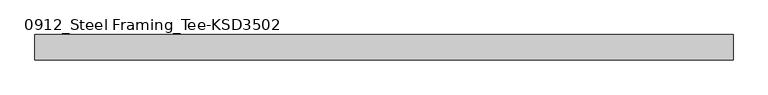
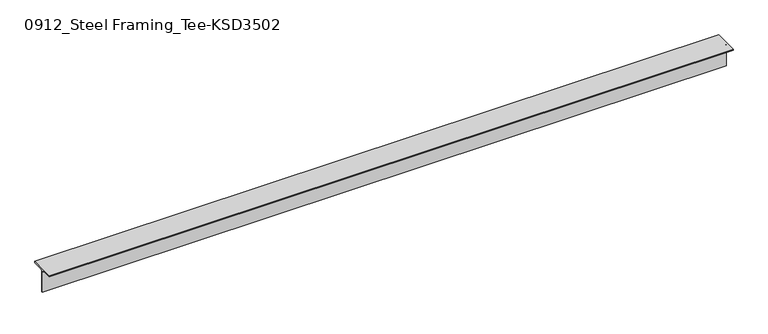
"""IFC4 building model written with IfcOpenShell, lengths in millimetres: member geometry, 0912_Steel Framing_Tee-KSD3502 : H_SB_ASB_CT-150x150x6.5x9."""

from ifc_helpers import new_model, si_unit, point, frame, frame_2d, origin, place, context, project, spatial, polyline, circle_curve, trimmed, segment, composite_curve, outline, extrude, source, transform, mapped, element, save


def member_0912_steel_framing_tee_ksd3502_323286f3(model_context):
    return source(origin(), model_context, "Body", "SweptSolid", [
        extrude(outline(composite_curve([segment(polyline([(-75.0, 75.0), (75.0, 75.0), (75.0, 66.0), (16.25, 66.0)]), True, "CONTINUOUS"), segment(trimmed(circle_curve(frame_2d((16.25, 53.0)), 13.0), [point((16.25, 66.0))], [point((3.25, 53.0))], True, "CARTESIAN"), True, "CONTINUOUS"), segment(polyline([(3.25, 53.0), (3.25, -75.0), (-3.25, -75.0), (-3.25, 53.0)]), True, "CONTINUOUS"), segment(trimmed(circle_curve(frame_2d((-16.25, 53.0)), 13.0), [point((-3.25, 53.0))], [point((-16.25, 66.0))], True, "CARTESIAN"), True, "CONTINUOUS"), segment(polyline([(-16.25, 66.0), (-75.0, 66.0), (-75.0, 75.0)]), True, "CONTINUOUS")], self_intersect=False)), frame((-2059.45, 0.0, 0.0), z_axis=(1.0, 0.0, 0.0), x_axis=(0.0, 1.0, 0.0)), (0.0, 0.0, 1.0), 4153.3),
    ])


if __name__ == "__main__":
    model = new_model("IFC4")
    model_context = context("Model", 3, world=origin())
    ifc_project = project(units=[si_unit("LENGTHUNIT", "METRE", prefix="MILLI")], contexts=[model_context])
    site = spatial("IfcSite", under=ifc_project)
    building = spatial("IfcBuilding", under=site)
    placement = place(None, origin())
    member_0912_steel_framing_tee_ksd3502_shape = member_0912_steel_framing_tee_ksd3502_323286f3(model_context)
    element("IfcMember", 1, ObjectType="0912_Steel Framing_Tee-KSD3502 : H_SB_ASB_CT-150x150x6.5x9", at=placement, inside=building, context=model_context, shape_type="MappedRepresentation", body=[
        mapped(member_0912_steel_framing_tee_ksd3502_shape, transform((0.0, 0.0, 0.0), x_axis=(1.0, 0.0, 0.0), y_axis=(0.0, 1.0, 0.0), z_axis=(0.0, 0.0, 1.0))),
    ])
    save(model, "model.ifc")

# Revit data of these elements
# Type "0912_Steel Framing_Tee-KSD3502 : H_SB_ASB_CT-150x150x6.5x9"
#   H_WM Code_1 = "S01AA003-00001 | Main Steel Structure Fabrication Work | Shelter/Building | Light Steel - Standard (30KG/M>Weight) | Material: (   )"
#   H_WM Code_2 = "S03AA029-00001 | Main Steel Structure Erection Work | Shelter/Building | Light Steel (30KG/M>Weight) | Material: (   )"
#   H_WM Code_3 = "S01AA010-00001 | Main Steel Structure Fabrication Work | Shelter/Building | Steel Painting/Coating | for Non-Fireproofed Steel Surface, Surface Preparation, Primer, Second & Final Coat | Material: (   )"
#   H_Q'ty Cal Type Tag = "SB-Q2"
#   Width = 15.0 cm
#   Web Thickness = 0.65 cm
#   Web Fillet = 1.3 cm
#   Section Area = 23.39 cm²
#   Perimeter = 0.60 m²/m
#   Nominal Weight = 18.40 kgf/m
#   Height = 15.0 cm
#   Flange Thickness = 0.9 cm
#   Centroid Vertical = 7.5 cm
#   Centroid Horizontal = 7.5 cm
#   Length [instance default] = 1.5000 m
#   Structural Material [instance default] = Steel, 45-345
#   Warping Constant = (empty or 0)
#   Torsional Moment of Inertia = 0
#   Section Name Key = ""
#   Plastic Modulus weak axis = 0
#   Plastic Modulus strong axis = 0
#   Moment of Inertia weak axis = 0
#   Moment of Inertia strong axis = 0
#   Elastic Modulus weak axis = 0
#   Elastic Modulus strong axis = 0
#   Bolt Spacing = 0
#   Assembly Code = ""
# Element 1 (IfcMember, "0912_Steel Framing_Tee-KSD3502 : H_SB_ASB_CT-150x150x6.5x9")
#   Structural Material = none
# Materials
#   "Steel, 45-345": class "Metal", colour RGB 189 187 185, transparency 0, Description = "Steel 345 MPa", Cost = 0
